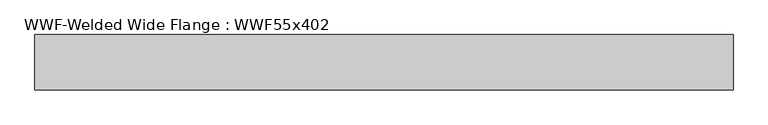
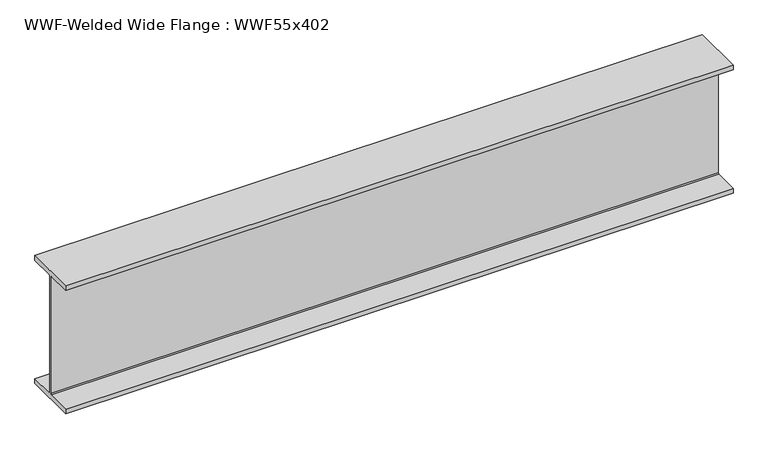
"""IFC4 building model written with IfcOpenShell, lengths in millimetres: beam geometry, WWF-Welded Wide Flange : WWF55x402."""

from ifc_helpers import new_model, si_unit, frame, origin, place, context, project, spatial, polyline, outline, extrude, source, transform, mapped, element, save


def wwf_welded_wide_flange_wwf55x402_ad15bced(model_context):
    return source(origin(), model_context, "Body", "SweptSolid", [
        extrude(outline(polyline([(274.955, -649.986), (274.955, -700.024), (-274.955, -700.024), (-274.955, -649.986), (-19.05, -649.986), (-8.001, -638.937), (-8.001, 638.937), (-19.05, 649.986), (-274.955, 649.986), (-274.955, 700.024), (274.955, 700.024), (274.955, 649.986), (19.05, 649.986), (8.001, 638.937), (8.001, -638.937), (19.05, -649.986), (274.955, -649.986)])), frame((-3459.52714, 0.0, 0.0), z_axis=(1.0, 0.0, 0.0), x_axis=(0.0, 1.0, 0.0)), (0.0, 0.0, 1.0), 6919.0542799),
    ])


if __name__ == "__main__":
    model = new_model("IFC4")
    model_context = context("Model", 3, world=origin())
    ifc_project = project(units=[si_unit("LENGTHUNIT", "METRE", prefix="MILLI")], contexts=[model_context])
    site = spatial("IfcSite", under=ifc_project)
    building = spatial("IfcBuilding", under=site)
    placement = place(None, origin())
    wwf_welded_wide_flange_wwf55x402_shape = wwf_welded_wide_flange_wwf55x402_ad15bced(model_context)
    element("IfcBeam", 1, ObjectType="WWF-Welded Wide Flange : WWF55x402", at=placement, inside=building, context=model_context, shape_type="MappedRepresentation", body=[
        mapped(wwf_welded_wide_flange_wwf55x402_shape, transform((0.0, 0.0, 0.0), x_axis=(1.0, 0.0, 0.0), y_axis=(0.0, 1.0, 0.0), z_axis=(0.0, 0.0, 1.0))),
    ])
    save(model, "model.ifc")

# Revit data of these elements
# Type "WWF-Welded Wide Flange : WWF55x402"
#   Assembly Code = "B10"
#   Nominal d = "12"
#   W = 402
#   Length [instance default] = 1524 mm
#   bf = 549.91 mm
#   d = 1400.048 mm
#   k = 19.05 mm
#   tf = 50.038 mm
#   tw = 16.002 mm
#   A = 0.0761289 m²
#   Structural Material [instance default] = Steel ASTM A572
# Element 1 (IfcBeam, "WWF-Welded Wide Flange : WWF55x402")
#   Structural Material = Metal - Steel 43-275
#   Materials on its faces: "Metal - Steel 43-275"
# Materials
#   "Steel ASTM A572": class "Metal", colour RGB 247 247 247, transparency 0, Description = "Structural steel, high strength low alloy, ASTM - A572 - 50", Cost = 0
#   "Metal - Steel 43-275": class "Metal", colour RGB 247 247 247, transparency 0, Cost = 0
